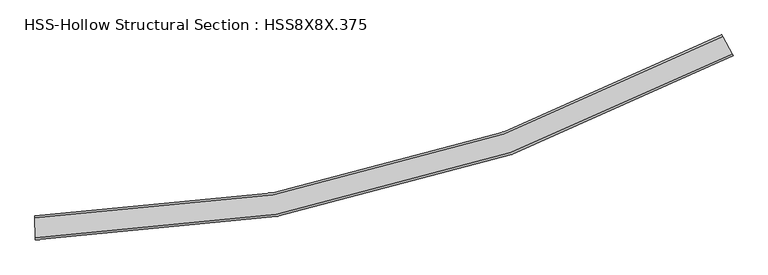
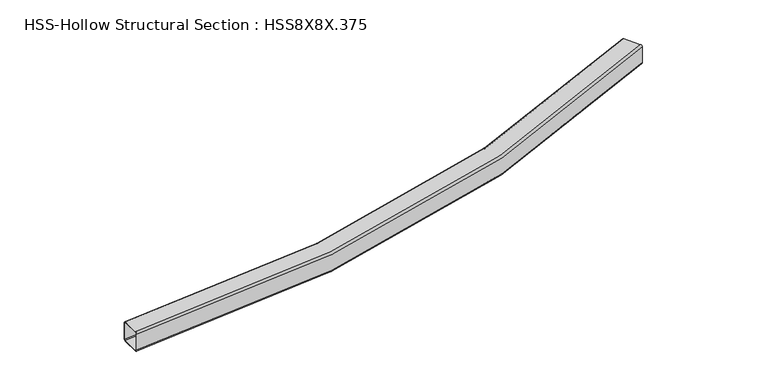
"""IFC4 building model written with IfcOpenShell, lengths in millimetres: beam geometry, HSS-Hollow Structural Section : HSS8X8X.375."""

from ifc_helpers import new_model, si_unit, point, frame, origin, place, context, project, spatial, polyline, circle_curve, ellipse_curve, trimmed, source, transform, mapped, element, save
from ifc_brep_helpers import plane_surface, cylinder_surface, revolved_surface, advanced_brep


def hss_hollow_structural_section_hss8x8x_375_31d8bada(model_context):
    return source(origin(), model_context, "Body", "AdvancedBrep", [
        advanced_brep(
        [(6121.7238156, 1466.3923014, 83.9390625), (6121.7238156, 1466.3923014, -83.9390625), (6113.2336242, 1481.8785974, -101.6), (6032.5291082, 1629.0854109, -101.6), (6024.0389168, 1644.5717069, -83.9390625), (6024.0389168, 1644.5717069, 83.9390625), (6032.5291082, 1629.0854109, 101.6), (6113.2336242, 1481.8785974, 101.6), (6032.5291082, 1629.0854109, 92.7695312), (6028.2840125, 1636.8285589, 83.9390625), (6028.2840125, 1636.8285589, -83.9390625), (6032.5291082, 1629.0854109, -92.7695313), (6113.2336242, 1481.8785974, -92.7695313), (6117.4787199, 1474.1354494, -83.9390625), (6117.4787199, 1474.1354494, 83.9390625), (6113.2336242, 1481.8785974, 92.7695312), (187.7413355, -100.2159767, 83.9390625), (187.4809579, -82.5569587, 101.6), (185.0059077, 85.3029203, 101.6), (184.7455301, 102.9619383, 83.9390625), (184.7455301, 102.9619383, -83.9390625), (185.0059077, 85.3029203, -101.6), (187.4809579, -82.5569587, -101.6), (187.7413355, -100.2159767, -83.9390625), (185.0059077, 85.3029203, 92.7695312), (187.4809579, -82.5569587, 92.7695312), (187.6111467, -91.3864677, 83.9390625), (187.6111467, -91.3864677, -83.9390625), (187.4809579, -82.5569587, -92.7695313), (185.0059077, 85.3029203, -92.7695313), (184.8757189, 94.1324293, -83.9390625), (184.8757189, 94.1324293, 83.9390625)],
        [
            (0, 1),
            (1, 2, circle_curve(frame((6113.2336242, 1481.8785974, -83.9390625), z_axis=(0.8768671529491879, 0.48073276992398356, 0.0), x_axis=(-0.48073276992398356, 0.8768671529491879, 0.0)), 17.6609375)),
            (2, 3),
            (3, 4, circle_curve(frame((6032.5291082, 1629.0854109, -83.9390625), z_axis=(0.8768671529491879, 0.48073276992398356, 0.0), x_axis=(-0.48073276992398356, 0.8768671529491879, 0.0)), 17.6609375)),
            (4, 5),
            (5, 6, circle_curve(frame((6032.5291082, 1629.0854109, 83.9390625), z_axis=(0.8768671529491879, 0.48073276992398356, 0.0), x_axis=(-0.48073276992398356, 0.8768671529491879, 0.0)), 17.6609375)),
            (6, 7),
            (7, 0, circle_curve(frame((6113.2336242, 1481.8785974, 83.9390625), z_axis=(0.8768671529491879, 0.48073276992398356, 0.0), x_axis=(-0.48073276992398356, 0.8768671529491879, 0.0)), 17.6609375)),
            (8, 9, circle_curve(frame((6032.5291082, 1629.0854109, 83.9390625), z_axis=(-0.8768671529491879, -0.48073276992398356, 0.0), x_axis=(-0.48073276992398356, 0.8768671529491879, 0.0)), 8.8304688)),
            (9, 10),
            (10, 11, circle_curve(frame((6032.5291082, 1629.0854109, -83.9390625), z_axis=(-0.8768671529491879, -0.48073276992398356, 0.0), x_axis=(-0.48073276992398356, 0.8768671529491879, 0.0)), 8.8304688)),
            (11, 12),
            (12, 13, circle_curve(frame((6113.2336242, 1481.8785974, -83.9390625), z_axis=(-0.8768671529491875, -0.4807327699239843, 0.0), x_axis=(-0.4807327699239843, 0.8768671529491875, 0.0)), 8.8304688)),
            (13, 14),
            (14, 15, circle_curve(frame((6113.2336242, 1481.8785974, 83.9390625), z_axis=(-0.8768671529491877, -0.4807327699239839, 0.0), x_axis=(-0.4807327699239839, 0.8768671529491877, 0.0)), 8.8304688)),
            (15, 8),
            (16, 17, circle_curve(frame((187.4809579, -82.5569587, 83.9390625), z_axis=(-0.999891314050926, -0.014743136895264575, 0.0), x_axis=(-0.014743136895264575, 0.999891314050926, 0.0)), 17.6609375)),
            (17, 18),
            (18, 19, circle_curve(frame((185.0059077, 85.3029203, 83.9390625), z_axis=(-0.999891314050926, -0.014743136895264575, 0.0), x_axis=(-0.014743136895264575, 0.999891314050926, 0.0)), 17.6609375)),
            (19, 20),
            (20, 21, circle_curve(frame((185.0059077, 85.3029203, -83.9390625), z_axis=(-0.999891314050926, -0.014743136895264575, 0.0), x_axis=(-0.014743136895264575, 0.999891314050926, 0.0)), 17.6609375)),
            (21, 22),
            (22, 23, circle_curve(frame((187.4809579, -82.5569587, -83.9390625), z_axis=(-0.999891314050926, -0.014743136895264575, 0.0), x_axis=(-0.014743136895264575, 0.999891314050926, 0.0)), 17.6609375)),
            (23, 16),
            (24, 25),
            (25, 26, circle_curve(frame((187.4809579, -82.5569587, 83.9390625), z_axis=(0.999891314050926, 0.014743136895264963, 0.0), x_axis=(-0.014743136895264963, 0.999891314050926, 0.0)), 8.8304688)),
            (26, 27),
            (27, 28, circle_curve(frame((187.4809579, -82.5569587, -83.9390625), z_axis=(0.999891314050926, 0.014743136895264963, 0.0), x_axis=(-0.014743136895264963, 0.999891314050926, 0.0)), 8.8304688)),
            (28, 29),
            (29, 30, circle_curve(frame((185.0059077, 85.3029203, -83.9390625), z_axis=(0.999891314050926, 0.014743136895264575, 0.0), x_axis=(-0.014743136895264575, 0.999891314050926, 0.0)), 8.8304688)),
            (30, 31),
            (31, 24, circle_curve(frame((185.0059077, 85.3029203, 83.9390625), z_axis=(0.999891314050926, 0.014743136895264575, 0.0), x_axis=(-0.014743136895264575, 0.999891314050926, 0.0)), 8.8304688)),
            (7, 17, circle_curve(frame((0.0, 12632.5512762, 101.6), z_axis=(0.0, 0.0, -1.0), x_axis=(-0.5014171979932397, 0.8652056365723748, 0.0)), 12716.4903387)),
            (16, 0, circle_curve(frame((0.0, 12632.5512762, 83.9390625), z_axis=(0.0, 0.0, 1.0), x_axis=(-0.5014171979932397, 0.8652056365723748, 0.0)), 12734.1512762)),
            (6, 18, circle_curve(frame((0.0, 12632.5512762, 101.6), z_axis=(0.0, 0.0, -1.0), x_axis=(-0.5014171979932397, 0.8652056365723748, 0.0)), 12548.6122137)),
            (5, 19, circle_curve(frame((0.0, 12632.5512762, 83.9390625), z_axis=(0.0, 0.0, -1.0), x_axis=(-0.5014171979932397, 0.8652056365723748, 0.0)), 12530.9512762)),
            (4, 20, circle_curve(frame((0.0, 12632.5512762, -83.9390625), z_axis=(0.0, 0.0, -1.0), x_axis=(-0.5014171979932397, 0.8652056365723748, 0.0)), 12530.9512762)),
            (3, 21, circle_curve(frame((0.0, 12632.5512762, -101.6), z_axis=(0.0, 0.0, -1.0), x_axis=(-0.5014171979932397, 0.8652056365723748, 0.0)), 12548.6122137)),
            (2, 22, circle_curve(frame((0.0, 12632.5512762, -101.6), z_axis=(0.0, 0.0, -1.0), x_axis=(-0.5014171979932397, 0.8652056365723748, 0.0)), 12716.4903387)),
            (1, 23, circle_curve(frame((0.0, 12632.5512762, -83.9390625), z_axis=(0.0, 0.0, -1.0), x_axis=(-0.5014171979932397, 0.8652056365723748, 0.0)), 12734.1512762)),
            (15, 25, circle_curve(frame((0.0, 12632.5512762, 92.7695312), z_axis=(0.0, 0.0, -1.0), x_axis=(-0.5014171979932397, 0.8652056365723748, 0.0)), 12716.4903387)),
            (24, 8, circle_curve(frame((0.0, 12632.5512762, 92.7695312), z_axis=(0.0, 0.0, 1.0), x_axis=(-0.5014171979932397, 0.8652056365723748, 0.0)), 12548.6122137)),
            (14, 26, circle_curve(frame((0.0, 12632.5512762, 83.9390625), z_axis=(0.0, 0.0, -1.0), x_axis=(-0.5014171979932397, 0.8652056365723748, 0.0)), 12725.3208075)),
            (13, 27, circle_curve(frame((0.0, 12632.5512762, -83.9390625), z_axis=(0.0, 0.0, -1.0), x_axis=(-0.5014171979932397, 0.8652056365723748, 0.0)), 12725.3208075)),
            (12, 28, circle_curve(frame((0.0, 12632.5512762, -92.7695313), z_axis=(0.0, 0.0, -1.0), x_axis=(-0.5014171979932397, 0.8652056365723748, 0.0)), 12716.4903387)),
            (11, 29, circle_curve(frame((0.0, 12632.5512762, -92.7695313), z_axis=(0.0, 0.0, -1.0), x_axis=(-0.5014171979932397, 0.8652056365723748, 0.0)), 12548.6122137)),
            (10, 30, circle_curve(frame((0.0, 12632.5512762, -83.9390625), z_axis=(0.0, 0.0, -1.0), x_axis=(-0.5014171979932397, 0.8652056365723748, 0.0)), 12539.781745)),
            (9, 31, circle_curve(frame((0.0, 12632.5512762, 83.9390625), z_axis=(0.0, 0.0, -1.0), x_axis=(-0.5014171979932397, 0.8652056365723748, 0.0)), 12539.781745)),
        ],
        [
            plane_surface(frame((6072.8813662, 1555.4820042, 0.0), z_axis=(0.8768671529491846, 0.4807327699239896, 0.0), x_axis=(0.0, 0.0, 1.0))),
            plane_surface(frame((186.2434328, 1.3729808, 0.0), z_axis=(-0.9998913140509259, -0.014743136895270903, 0.0), x_axis=(0.0, 0.0, 1.0))),
            revolved_surface(trimmed(ellipse_curve(frame((-6376.2669539, 23634.9303947, 83.9390625), z_axis=(-0.8652056365723783, -0.5014171979932338, 0.0), x_axis=(0.5014171979932338, -0.8652056365723783, 0.0)), 17.6609375, 17.6609375), [point((-6376.2669539, 23634.9303947, 101.6))], [point((-6385.1224517, 23650.2107374, 83.9390625))], True, "CARTESIAN"), (0.0, 12632.5512762, 0.0), (0.0, 0.0, -1.0)),
            plane_surface(frame((0.0, 12632.5512762, 101.6), z_axis=(0.0, 0.0, 1.0), x_axis=(-0.5014171979932397, 0.8652056365723748, 0.0))),
            revolved_surface(trimmed(ellipse_curve(frame((-6292.0899749, 23489.6812947, 83.9390625), z_axis=(-0.8652056365723783, -0.5014171979932338, 0.0), x_axis=(0.5014171979932338, -0.8652056365723783, 0.0)), 17.6609375, 17.6609375), [point((-6283.2344771, 23474.400952, 83.9390625))], [point((-6292.0899749, 23489.6812947, 101.6))], True, "CARTESIAN"), (0.0, 12632.5512762, 0.0), (0.0, 0.0, -1.0)),
            revolved_surface(polyline([(-6283.234477102014, 23474.400951982032, -83.9390625), (-6283.234477102014, 23474.400951982032, 83.9390625)]), (0.0, 12632.5512762, 0.0), (0.0, 0.0, -1.0)),
            revolved_surface(trimmed(ellipse_curve(frame((-6292.0899749, 23489.6812947, -83.9390625), z_axis=(-0.8652056365723783, -0.5014171979932338, 0.0), x_axis=(0.5014171979932338, -0.8652056365723783, 0.0)), 17.6609375, 17.6609375), [point((-6292.0899749, 23489.6812947, -101.6))], [point((-6283.2344771, 23474.400952, -83.9390625))], True, "CARTESIAN"), (0.0, 12632.5512762, 0.0), (0.0, 0.0, -1.0)),
            plane_surface(frame((0.0, 12632.5512762, -101.6), z_axis=(0.0, 0.0, -1.0), x_axis=(-0.5014171979932397, 0.8652056365723748, 0.0))),
            revolved_surface(trimmed(ellipse_curve(frame((-6376.2669539, 23634.9303947, -83.9390625), z_axis=(-0.8652056365723783, -0.5014171979932338, 0.0), x_axis=(0.5014171979932338, -0.8652056365723783, 0.0)), 17.6609375, 17.6609375), [point((-6385.1224517, 23650.2107374, -83.9390625))], [point((-6376.2669539, 23634.9303947, -101.6))], True, "CARTESIAN"), (0.0, 12632.5512762, 0.0), (0.0, 0.0, -1.0)),
            cylinder_surface(frame((0.0, 12632.5512762, 0.0), z_axis=(0.0, 0.0, -1.0), x_axis=(-0.5014171979932397, 0.8652056365723748, 0.0)), 12734.1512762),
            plane_surface(frame((0.0, 12632.5512762, 92.7695312), z_axis=(0.0, 0.0, -1.0), x_axis=(-0.5014171979932397, 0.8652056365723748, 0.0))),
            revolved_surface(trimmed(ellipse_curve(frame((-6376.2669539, 23634.9303947, 83.9390625), z_axis=(0.865205636572378, 0.5014171979932341, 0.0), x_axis=(0.5014171979932341, -0.865205636572378, 0.0)), 8.8304688, 8.8304688), [point((-6380.6947028, 23642.570566, 83.9390625))], [point((-6376.2669539, 23634.9303947, 92.7695312))], True, "CARTESIAN"), (0.0, 12632.5512762, 0.0), (0.0, 0.0, -1.0)),
            revolved_surface(polyline([(-6380.6947028617205, 23642.570566040726, -83.9390625), (-6380.6947028617205, 23642.570566040726, 83.9390625)]), (0.0, 12632.5512762, 0.0), (0.0, 0.0, -1.0)),
            revolved_surface(trimmed(ellipse_curve(frame((-6376.2669539, 23634.9303947, -83.9390625), z_axis=(0.865205636572378, 0.5014171979932341, 0.0), x_axis=(0.5014171979932341, -0.865205636572378, 0.0)), 8.8304688, 8.8304688), [point((-6376.2669539, 23634.9303947, -92.7695313))], [point((-6380.6947028, 23642.570566, -83.9390625))], True, "CARTESIAN"), (0.0, 12632.5512762, 0.0), (0.0, 0.0, -1.0)),
            plane_surface(frame((0.0, 12632.5512762, -92.7695313), z_axis=(0.0, 0.0, 1.0), x_axis=(-0.5014171979932397, 0.8652056365723748, 0.0))),
            revolved_surface(trimmed(ellipse_curve(frame((-6292.0899749, 23489.6812947, -83.9390625), z_axis=(0.8652056365723783, 0.5014171979932338, 0.0), x_axis=(0.5014171979932338, -0.8652056365723783, 0.0)), 8.8304688, 8.8304688), [point((-6287.662226, 23482.0411234, -83.9390625))], [point((-6292.0899749, 23489.6812947, -92.7695313))], True, "CARTESIAN"), (0.0, 12632.5512762, 0.0), (0.0, 0.0, -1.0)),
            cylinder_surface(frame((0.0, 12632.5512762, 0.0), z_axis=(0.0, 0.0, -1.0), x_axis=(-0.5014171979932397, 0.8652056365723748, 0.0)), 12539.781745),
            revolved_surface(trimmed(ellipse_curve(frame((-6292.0899749, 23489.6812947, 83.9390625), z_axis=(0.8652056365723783, 0.5014171979932338, 0.0), x_axis=(0.5014171979932338, -0.8652056365723783, 0.0)), 8.8304688, 8.8304688), [point((-6292.0899749, 23489.6812947, 92.7695312))], [point((-6287.662226, 23482.0411234, 83.9390625))], True, "CARTESIAN"), (0.0, 12632.5512762, 0.0), (0.0, 0.0, -1.0)),
        ],
        [
            (0, [[1, 2, 3, 4, 5, 6, 7, 8], [9, 10, 11, 12, 13, 14, 15, 16]]),
            (1, [[17, 18, 19, 20, 21, 22, 23, 24], [25, 26, 27, 28, 29, 30, 31, 32]]),
            (2, [[33, -17, 34, -8]]),
            (3, [[35, -18, -33, -7]]),
            (4, [[36, -19, -35, -6]]),
            (5, [[37, -20, -36, -5]]),
            (6, [[38, -21, -37, -4]]),
            (7, [[39, -22, -38, -3]]),
            (8, [[40, -23, -39, -2]]),
            (9, [[-34, -24, -40, -1]]),
            (10, [[41, -25, 42, -16]]),
            (11, [[43, -26, -41, -15]]),
            (12, [[44, -27, -43, -14]]),
            (13, [[45, -28, -44, -13]]),
            (14, [[46, -29, -45, -12]]),
            (15, [[47, -30, -46, -11]]),
            (16, [[48, -31, -47, -10]]),
            (17, [[-42, -32, -48, -9]]),
        ],
    ),
    ])


if __name__ == "__main__":
    model = new_model("IFC4")
    model_context = context("Model", 3, world=origin())
    ifc_project = project(units=[si_unit("LENGTHUNIT", "METRE", prefix="MILLI")], contexts=[model_context])
    site = spatial("IfcSite", under=ifc_project)
    building = spatial("IfcBuilding", under=site)
    placement = place(None, origin())
    hss_hollow_structural_section_hss8x8x_375_shape = hss_hollow_structural_section_hss8x8x_375_31d8bada(model_context)
    element("IfcBeam", 1, ObjectType="HSS-Hollow Structural Section : HSS8X8X.375", at=placement, inside=building, context=model_context, shape_type="MappedRepresentation", body=[
        mapped(hss_hollow_structural_section_hss8x8x_375_shape, transform((0.0, 0.0, 0.0), x_axis=(1.0, 0.0, 0.0), y_axis=(0.0, 1.0, 0.0), z_axis=(0.0, 0.0, 1.0))),
    ])
    save(model, "model.ifc")

# Revit data of these elements
# Type "HSS-Hollow Structural Section : HSS8X8X.375"
#   Assembly Code = "B10"
#   Shape = "Square"
#   W = 37.6
#   Start Extension Calculation [instance default] = 10' - 0"
#   Start Extension [instance default] = -0' - 0 1/2"
#   End Extension Calculation [instance default] = 10' - 0"
#   End Extension [instance default] = -0' - 0 1/2"
#   Ht = 0' - 8"
#   Length [instance default] = 5' - 0"
#   b = 0' - 8"
#   kr = 0' - 0 89/128"
#   t = 0' - 0 89/256"
#   A = 0.0722222 SF
#   Beam Material [instance default] = Metal - Steel - ASTM A500 - Grade B - Rectangular and Square
# Element 1 (IfcBeam, "HSS-Hollow Structural Section : HSS8X8X.375")
#   Materials on its faces: "Metal - Steel - ASTM A500 - Grade B - Rectangular and Square"
# Materials
#   "Metal - Steel - ASTM A500 - Grade B - Rectangular and Square": class "Metal", colour RGB 128 0 0, transparency 0
